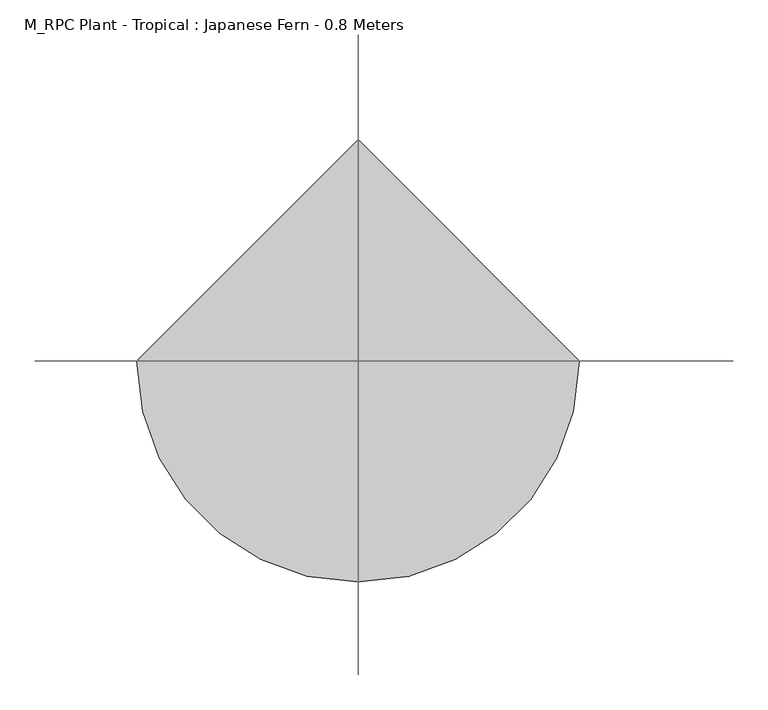
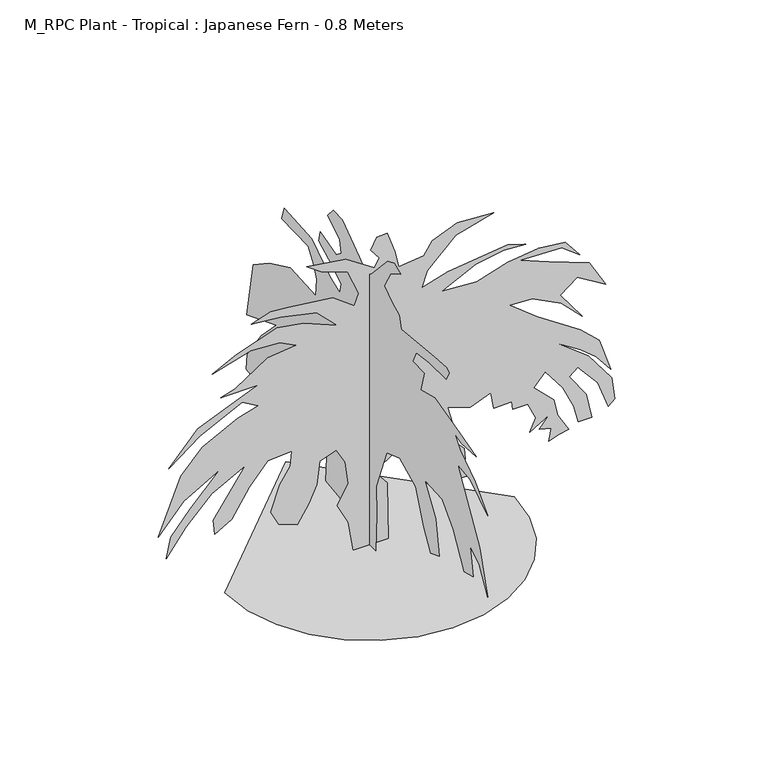
"""IFC4 building model written with IfcOpenShell, lengths in millimetres: geographic element geometry, M_RPC Plant - Tropical : Japanese Fern - 0.8 Meters."""

import ifcopenshell
import ifcopenshell.guid

model = None  # the IFC model being written
_history = None  # IfcOwnerHistory: only IFC2X3 demands one
_inside = {}  # id of a spatial element -> (the spatial element, [elements in it])
_under = {}  # id of a project, library or spatial element -> (it, [spatial elements below it])
_declared = {}  # id of a project -> (the project, [libraries it declares])
_typed = {}  # id of a type object -> (the type object, [elements of that type])
_made_of = {}  # id of a material, layer set ... -> (it, [elements and type objects made of it])


def new_model(schema):
    """Start an empty IFC model of exactly this schema.

    Asked for "IFC4X3", IfcOpenShell would pick the latest addendum, in which some entities
    have other attributes; the version numbers below select the first issue.
    IFC2X3 requires an IfcOwnerHistory on every rooted entity: one is made here for all.
    """
    global model, _history
    if schema == "IFC4X3":
        model = ifcopenshell.file(schema_version=(4, 3, 0, 0))
    else:
        model = ifcopenshell.file(schema=schema)
    _inside.clear()
    _under.clear()
    _declared.clear()
    _typed.clear()
    _made_of.clear()
    _history = None
    if model.schema == "IFC2X3":
        org = make("IfcOrganization", Name="unknown")
        user = make(
            "IfcPersonAndOrganization",
            ThePerson=make("IfcPerson", FamilyName="unknown"),
            TheOrganization=org,
        )
        app = make(
            "IfcApplication",
            ApplicationDeveloper=org,
            Version="unknown",
            ApplicationFullName="unknown",
            ApplicationIdentifier="unknown",
        )
        _history = make(
            "IfcOwnerHistory",
            OwningUser=user,
            OwningApplication=app,
            ChangeAction="ADDED",
            CreationDate=0,
        )
    return model


def make(cls, **values):
    """One entity of the class cls with the attributes given. An attribute that is None is left unset."""
    return model.create_entity(
        cls, **{name: value for name, value in values.items() if value is not None}
    )


def rooted(cls, **values):
    """An entity with a GlobalId (a new one), such as an element, a storey or a relation."""
    return make(cls, GlobalId=ifcopenshell.guid.new(), OwnerHistory=_history, **values)


def si_unit(unit_type, name, prefix=None):
    """IfcSIUnit, for example si_unit("LENGTHUNIT", "METRE", prefix="MILLI")."""
    return make("IfcSIUnit", UnitType=unit_type, Prefix=prefix, Name=name)


def assignment(units):
    """IfcUnitAssignment: the units of a project."""
    return None if units is None else make("IfcUnitAssignment", Units=units)


def point(xyz):
    """IfcCartesianPoint."""
    return None if xyz is None else make("IfcCartesianPoint", Coordinates=xyz)


def direction(xyz):
    """IfcDirection."""
    return None if xyz is None else make("IfcDirection", DirectionRatios=xyz)


def frame(location, z_axis=None, x_axis=None):
    """IfcAxis2Placement3D, a coordinate frame: its origin and axes. An axis left out is left unset."""
    return make(
        "IfcAxis2Placement3D",
        Location=point(location),
        Axis=direction(z_axis),
        RefDirection=direction(x_axis),
    )


def origin():
    """The frame at (0, 0, 0) with its axes left unset."""
    return frame((0.0, 0.0, 0.0))


def place(relative_to, where):
    """IfcLocalPlacement: puts the frame where relative to a parent placement (None: the world)."""
    return make(
        "IfcLocalPlacement", PlacementRelTo=relative_to, RelativePlacement=where
    )


def context(
    kind, dimensions, precision=None, world=None, true_north=None, identifier=None
):
    """IfcGeometricRepresentationContext, for example the 3D "Model" context."""
    return make(
        "IfcGeometricRepresentationContext",
        ContextIdentifier=identifier,
        ContextType=kind,
        CoordinateSpaceDimension=dimensions,
        Precision=precision,
        WorldCoordinateSystem=world,
        TrueNorth=true_north,
    )


def project(units=None, contexts=None):
    """IfcProject with its units and contexts."""
    return rooted(
        "IfcProject",
        Name="project",
        RepresentationContexts=contexts,
        UnitsInContext=assignment(units),
    )


def spatial(cls, under=None, at=None, **own):
    """A site, building, storey or space (cls), placed at a placement, below another one or the project."""
    s = rooted(cls, ObjectPlacement=at, **own)
    if under is not None:
        _under.setdefault(under.id(), (under, []))[1].append(s)
    return s


def point_list(points):
    """IfcCartesianPointList2D or 3D."""
    cls = (
        "IfcCartesianPointList2D" if len(points[0]) == 2 else "IfcCartesianPointList3D"
    )
    return make(cls, CoordList=points)


def triangles(points, corners, closed=None, point_numbers=None):
    """IfcTriangulatedFaceSet: each triangle names its three corners, points numbered from 1."""
    return make(
        "IfcTriangulatedFaceSet",
        Coordinates=point_list(points),
        Closed=closed,
        CoordIndex=corners,
        PnIndex=point_numbers,
    )


def shape(context_of_items, identifier, shape_type, items):
    """IfcShapeRepresentation: the items that make up one representation, for example the "Body"."""
    return make(
        "IfcShapeRepresentation",
        ContextOfItems=context_of_items,
        RepresentationIdentifier=identifier,
        RepresentationType=shape_type,
        Items=items,
    )


def source(mapping_origin, context_of_items, identifier, shape_type, items):
    """IfcRepresentationMap: a shape defined once, which mapped items show again and again."""
    return make(
        "IfcRepresentationMap",
        MappingOrigin=mapping_origin,
        MappedRepresentation=shape(context_of_items, identifier, shape_type, items),
    )


def transform(
    local_origin,
    x_axis=None,
    y_axis=None,
    z_axis=None,
    scale=None,
    scale2=None,
    scale3=None,
    uniform=True,
):
    """IfcCartesianTransformationOperator3D, or its non-uniform kind. x_axis, y_axis, z_axis: its Axis1, 2, 3."""
    if uniform:
        return make(
            "IfcCartesianTransformationOperator3D",
            Axis1=direction(x_axis),
            Axis2=direction(y_axis),
            LocalOrigin=point(local_origin),
            Scale=scale,
            Axis3=direction(z_axis),
        )
    return make(
        "IfcCartesianTransformationOperator3DnonUniform",
        Axis1=direction(x_axis),
        Axis2=direction(y_axis),
        LocalOrigin=point(local_origin),
        Scale=scale,
        Axis3=direction(z_axis),
        Scale2=scale2,
        Scale3=scale3,
    )


def mapped(mapping_source, mapping_target):
    """IfcMappedItem: shows the shape of a source again, moved by a transform."""
    return make(
        "IfcMappedItem", MappingSource=mapping_source, MappingTarget=mapping_target
    )


def made_of(thing, what):
    """Note that an element or type object is made of a material, layer set ...; save() writes the relation."""
    if what is not None:
        _made_of.setdefault(what.id(), (what, []))[1].append(thing)
    return thing


def element(
    cls,
    number,
    at=None,
    inside=None,
    cuts=None,
    type_object=None,
    material=None,
    context=None,
    identifier="Body",
    shape_type=None,
    held_by="IfcProductDefinitionShape",
    body=None,
    shapes=None,
    **own,
):
    """One element of the class cls, such as IfcWall. Its Tag is "e" and its number.

    at: its placement. inside: the storey or other place that contains it. cuts: it is an
    opening in that element (IfcRelVoidsElement). A single representation is given by context,
    identifier, shape_type and body (its items); several are given by shapes. held_by: the class
    of the entity that holds the representations. save() writes the other relations.
    """
    e = rooted(cls, Tag="e%d" % number, ObjectPlacement=at, **own)
    if body is not None:
        shapes = [shape(context, identifier, shape_type, body)]
    if shapes is not None:
        e.Representation = make(held_by, Representations=shapes)
    if inside is not None:
        _inside.setdefault(inside.id(), (inside, []))[1].append(e)
    if cuts is not None:
        rooted(
            "IfcRelVoidsElement", RelatingBuildingElement=cuts, RelatedOpeningElement=e
        )
    if type_object is not None:
        _typed.setdefault(type_object.id(), (type_object, []))[1].append(e)
    return made_of(e, material)


def aggregate(whole, parts):
    """IfcRelAggregates: a whole, such as a stair, and the parts it consists of."""
    return rooted("IfcRelAggregates", RelatingObject=whole, RelatedObjects=parts)


def save(model, path):
    """Write the relations noted so far, then the file.

    IfcRelAggregates (storeys below a building ...), IfcRelContainedInSpatialStructure (elements
    in a storey), IfcRelDefinesByType, IfcRelAssociatesMaterial and IfcRelDeclares: one each for
    every whole, place, type object, material and project.
    """
    for whole, parts in _under.values():
        aggregate(whole, parts)
    for where, things in _inside.values():
        rooted(
            "IfcRelContainedInSpatialStructure",
            RelatedElements=things,
            RelatingStructure=where,
        )
    for kind, things in _typed.values():
        rooted("IfcRelDefinesByType", RelatedObjects=things, RelatingType=kind)
    for what, things in _made_of.values():
        rooted("IfcRelAssociatesMaterial", RelatedObjects=things, RelatingMaterial=what)
    for by, libraries in _declared.values():
        rooted("IfcRelDeclares", RelatingContext=by, RelatedDefinitions=libraries)
    model.write(path)


def m_rpc_plant_tropical_japanese_fern_0_8_meters_89f61e38(model_context):
    return source(origin(), model_context, "Body", "Tessellation", [
        triangles([(-356.9816259, 0.0, 2.46e-05), (-347.538961, -81.8417886, 2.46e-05), (-320.6483422, -157.0003733, 2.46e-05), (-278.4590569, -223.3224515, 2.46e-05), (-223.1257884, -278.6557201, 2.46e-05), (-156.8037101, -320.8450235, 2.46e-05), (-81.6451164, -347.7356423, 2.46e-05), (0.1966867, -357.1783072, 2.46e-05), (82.0384609, -347.7356423, 2.46e-05), (157.1970364, -320.8450235, 2.46e-05), (223.5191146, -278.6557201, 2.46e-05), (278.8523832, -223.3224515, 2.46e-05), (321.0417048, -157.0003733, 2.46e-05), (347.9323236, -81.8417886, 2.46e-05), (357.3749886, 3.12e-05, 2.46e-05), (0.1966242, 357.1783072, 2.46e-05), (-39.591288, 2.4e-05, 3.8e-06), (-52.3886082, 2.53e-05, 77.2092589), (-79.4701856, 2.33e-05, 129.9044073), (-51.8286088, 1.92e-05, 179.0246285), (-59.6237998, 1.61e-05, 237.2005651), (-81.0099172, 1.47e-05, 275.3224025), (-121.8640096, 1.74e-05, 260.7322683), (-129.4650627, 2.12e-05, 202.3781994), (-150.0026445, 2.47e-05, 159.3985009), (-177.3082362, 2.85e-05, 114.8257492), (-224.1652416, 2.95e-05, 132.5502668), (-243.9444304, 2.81e-05, 171.1790318), (-221.0799103, 2.33e-05, 234.4691003), (-195.0511394, 1.98e-05, 273.6130591), (-191.2119478, 1.74e-05, 311.3276902), (-250.2614867, 2.02e-05, 307.4210246), (-296.6350369, 2.54e-05, 254.2280142), (-339.5123071, 3.14e-05, 185.9592888), (-381.4722822, 3.47e-05, 161.1515734), (-385.2696158, 3.25e-05, 199.7619347), (-305.7070304, 2.23e-05, 313.25835), (-389.2322737, 2.86e-05, 269.5890678), (-451.6135314, 3.51e-05, 205.2877965), (-501.5068159, 4.12e-05, 139.8979924), (-490.5788492, 3.76e-05, 191.9816683), (-441.6242065, 3.21e-05, 249.0544201), (-368.8616057, 2.43e-05, 325.6103577), (-458.3148665, 3.13e-05, 274.3943886), (-521.6481374, 3.83e-05, 202.3696607), (-465.4295122, 2.75e-05, 342.7516442), (-412.306919, 2.18e-05, 399.0182679), (-325.1523188, 1.53e-05, 444.1942168), (-273.6057376, 1.22e-05, 459.1648873), (-314.0723265, 1.26e-05, 482.4155394), (-418.6162359, 2.03e-05, 430.012924), (-495.2054927, 2.71e-05, 372.3782879), (-423.1042251, 1.92e-05, 451.5675676), (-315.4003341, 1.18e-05, 496.7035117), (-275.4804052, 9.1e-06, 512.7808371), (-366.2136206, 1.31e-05, 512.5835017), (-331.2056557, 1.09e-05, 523.2341598), (-250.2614867, 4.2e-06, 575.8901027), (-180.8079499, 7e-07, 584.7194329), (-221.0799103, 1.2e-06, 605.0713883), (-292.4937199, 4.1e-06, 609.4207232), (-387.4135983, 9.9e-06, 581.7274281), (-328.4856545, 5.5e-06, 612.0154049), (-227.295374, -1e-06, 646.7967121), (-161.5869029, -3.2e-06, 635.7193359), (-78.621382, -4.8e-06, 600.674055), (-129.4533356, -5.6e-06, 651.5887161), (-219.3260566, -2.8e-06, 670.7326784), (-291.1150432, -1e-07, 678.0232944), (-243.6241556, -3.1e-06, 694.5326792), (-199.2876722, -4.8e-06, 690.5139565), (-89.7989701, -8.8e-06, 676.7513517), (-37.2379591, -8.7e-06, 637.1700468), (-25.5654385, -1.1e-05, 666.3513325), (-53.2067405, -1.36e-05, 730.9165775), (-118.8594782, -1.21e-05, 754.0578976), (-153.9631858, -1.22e-05, 780.1592113), (-58.1566019, -1.55e-05, 766.6525503), (12.3701786, -1.58e-05, 718.8793036), (24.5030987, -1.76e-05, 741.3032982), (3.6158409, -1.84e-05, 768.4872494), (18.7047597, -2.07e-05, 796.1618683), (43.7640938, -2.19e-05, 798.4898512), (62.816342, -1.95e-05, 744.3539114), (72.129132, -1.74e-05, 701.4126371), (134.0245409, -2.04e-05, 707.8552671), (155.3583768, -2.33e-05, 739.3059637), (216.6393747, -2.75e-05, 765.5672241), (307.1003683, -3.11e-05, 759.7325512), (213.1465828, -2.54e-05, 733.5272467), (143.1669335, -1.83e-05, 665.9780268), (130.1258781, -1.53e-05, 625.1620588), (193.29407, -1.93e-05, 645.9246723), (342.1190157, -2.69e-05, 663.433996), (386.0096143, -2.8e-05, 650.2686659), (331.6310294, -2.58e-05, 653.215361), (262.3572055, -2.2e-05, 640.2313425), (179.4618111, -1.6e-05, 599.1567421), (265.035058, -1.94e-05, 594.3860667), (342.0896934, -2.42e-05, 617.5967503), (417.9909471, -2.81e-05, 628.4153486), (483.3268573, -3.05e-05, 620.5620489), (520.1241752, -2.95e-05, 575.8901027), (475.7348788, -2.95e-05, 609.4687217), (372.9456588, -2.52e-05, 612.3860945), (441.3349073, -2.65e-05, 584.6447645), (542.8041498, -2.87e-05, 546.4048021), (584.2227699, -2.63e-05, 476.0742113), (513.9028253, -2.58e-05, 519.0714778), (472.0308898, -2.2e-05, 486.8048427), (525.9615005, -2e-05, 412.4742416), (473.4335295, -2.08e-05, 465.0022127), (402.3962957, -1.99e-05, 501.5674953), (346.6470097, -1.76e-05, 504.9195073), (415.0709218, -1.74e-05, 450.4102255), (520.5801793, -1.78e-05, 379.9196154), (568.2414416, -1.72e-05, 335.1356847), (596.0814211, -1.33e-05, 249.2213612), (560.7561427, -1.45e-05, 294.909034), (522.6121774, -1.47e-05, 326.2076686), (462.342891, -1.43e-05, 363.9543108), (540.550799, -1.42e-05, 304.5037063), (599.2467439, -1.21e-05, 226.7565805), (605.6067481, -9e-06, 169.6256927), (590.1587448, -7.5e-06, 155.6795782), (563.8974481, -1.05e-05, 225.714711), (514.2895022, -1.18e-05, 284.0770462), (493.1588516, -9.9e-06, 266.7677284), (536.2361641, -8.1e-06, 205.2771322), (549.3054608, -4.8e-06, 141.0889262), (516.425491, -3.3e-06, 140.2646579), (505.3241701, -5.5e-06, 185.108614), (477.6415575, -7.8e-06, 243.2032329), (434.3535748, -9.2e-06, 299.3437015), (405.9722766, -6.1e-06, 268.3197412), (455.9268946, -5.4e-06, 219.8784575), (465.4788915, -3.2e-06, 174.9152863), (492.2202098, -1.7e-06, 130.1460077), (468.8415496, -3e-07, 124.1884135), (442.7215596, 1.3e-06, 116.1070845), (449.5455617, -8e-07, 146.8782531), (419.662938, 0.0, 155.0435705), (444.2522438, -2.8e-06, 184.860882), (396.2229444, 1e-06, 156.0027779), (410.9322573, -1.6e-06, 188.0872839), (391.7616251, -3.2e-06, 229.804832), (353.6443296, -1.6e-06, 230.0109786), (351.7750033, -2.7e-06, 250.1848198), (307.1003683, -7e-07, 249.0597613), (300.2817075, -2.9e-06, 291.6023862), (248.7385418, 5e-07, 272.405066), (193.29407, 1.9e-06, 289.9143715), (210.8028487, 4.9e-06, 225.714711), (209.5596469, 6.7e-06, 196.5163297), (234.147899, 7.2e-06, 170.2702392), (237.0660348, 8.8e-06, 141.0889262), (219.1519212, 1.04e-05, 127.6382756), (249.9017521, 1.1e-05, 94.9585752), (191.3132679, 1.34e-05, 97.4711035), (201.263133, 1.05e-05, 139.9955973), (173.9058276, 1.05e-05, 159.8089046), (182.4415529, 8.6e-06, 185.1459482), (114.684288, 1.2e-05, 178.0643492), (99.9141775, 1.12e-05, 202.3696607), (152.4405135, 7.1e-06, 231.5509645), (87.6747175, 9.8e-06, 234.8944377), (12.4554318, 1.6e-05, 186.0566121), (44.4696966, 1.69e-05, 146.9251888), (47.3878233, 1.91e-05, 0.0), (0.1988968, 28.0250381, 3.7e-06), (0.1989024, 23.3153101, 131.4809371), (0.1989043, 63.1703357, 135.2526637), (0.1989031, 125.3580096, 45.104755), (0.1989061, 186.8720783, 53.6724779), (0.1989088, 182.1083611, 118.7774792), (0.1989112, 144.4259864, 212.5160617), (0.1989072, 143.3849253, 265.1541278), (0.1989091, 175.7563505, 275.9837175), (0.1989147, 237.6858916, 199.7619347), (0.198915, 302.7357001, 140.1214617), (0.1989165, 331.3730146, 147.3601187), (0.1989186, 325.3463476, 199.5424713), (0.1989213, 363.9222997, 223.1101825), (0.1989223, 429.8262348, 180.7067569), (0.1989222, 475.8741872, 131.4809371), (0.1989247, 526.6901261, 139.4206596), (0.1989263, 521.9248283, 180.7067569), (0.1989212, 463.1728912, 264.866936), (0.1989213, 397.7889462, 332.7090159), (0.1989246, 523.5141572, 283.9223863), (0.1989299, 495.7835097, 430.9862294), (0.1989289, 428.236906, 476.0608764), (0.1989268, 339.3143177, 517.3488358), (0.1989217, 228.4952462, 512.2821756), (0.1989235, 224.9824519, 557.0447777), (0.1989254, 238.2328241, 586.9834299), (0.198928, 261.7722666, 621.3780602), (0.198933, 375.8342906, 623.7380178), (0.198934, 364.7196347, 657.0846743), (0.1989285, 247.1213622, 649.612674), (0.1989229, 169.3534347, 598.4660866), (0.1989203, 125.6708085, 581.7007582), (0.1989213, 121.2033486, 608.4554114), (0.1989249, 174.1686204, 639.6180079), (0.1989278, 217.0427113, 661.8500084), (0.1989224, 209.1029888, 690.4313307), (0.1989186, 140.9505263, 671.9353666), (0.1989184, 120.1790834, 688.8446543), (0.1989201, 126.4332074, 719.3166315), (0.1989238, 178.9323558, 752.3619255), (0.1989239, 155.1134427, 779.3565714), (0.1989222, 117.0030872, 777.7672062), (0.1989167, 43.7690217, 725.5806387), (0.1989142, 11.282335, 699.1806513), (0.1989139, -10.6222293, 714.4366241), (0.1989141, -78.3121894, 787.2951857), (0.1989134, -106.8948288, 799.9992067), (0.1989117, -133.8897381, 787.2951857), (0.1989124, -91.4905729, 762.6498877), (0.1989115, -63.82447, 714.9192982), (0.198909, -97.1412363, 690.3886734), (0.1989071, -127.8788042, 676.3806622), (0.1989116, -136.2243976, 645.8900087), (0.1988998, -278.3917282, 660.2606432), (0.1988976, -330.7943436, 663.4366848), (0.1988968, -341.9089994, 655.4979979), (0.1989026, -329.2050147, 631.6793936), (0.1989057, -255.7989394, 630.9247158), (0.1989078, -201.4115251, 623.4394169), (0.1989071, -185.4035451, 591.3727332), (0.1989049, -234.4786928, 590.4820899), (0.1989033, -219.4389858, 537.8608106), (0.1989013, -279.9783864, 553.8714612), (0.1988956, -384.8262926, 526.9594774), (0.1988915, -456.2395572, 506.2314912), (0.1988942, -394.0155936, 503.9995053), (0.1988957, -365.7943148, 511.6901696), (0.1988935, -388.4636069, 482.6261733), (0.1988888, -452.284893, 439.6635704), (0.198884, -507.0528437, 383.9622828), (0.1988894, -430.8768974, 431.8128868), (0.198892, -378.3489627, 438.6928811), (0.1988872, -418.3222495, 368.7036212), (0.1988809, -472.1195472, 279.1570521), (0.1988809, -505.8634904, 170.2702392), (0.198879, -470.530182, 233.1083004), (0.1988817, -430.9435721, 256.6434736), (0.1988781, -444.5382365, 186.5443548), (0.1988855, -406.6475987, 176.1064927), (0.198885, -359.3756295, 258.5152162), (0.1988892, -311.2476806, 308.3676965), (0.1988927, -237.3971011, 313.25835), (0.1988874, -284.7437206, 241.0480229), (0.1988892, -298.5170441, 151.7734485), (0.1988901, -261.8053315, 136.5182659), (0.1988937, -232.8570984, 188.3064747), (0.1988926, -197.5672648, 272.0370652), (0.198897, -130.1718691, 304.5676922), (0.1988986, -73.5660583, 284.6663815), (0.1989018, -28.8695723, 170.457437), (0.1988986, -31.953834, 99.3204365), (0.1988944, -26.9829074, 2.55e-05)], [[15, 16, 1], [14, 15, 1], [14, 1, 2], [13, 14, 2], [13, 2, 3], [13, 3, 4], [12, 13, 4], [11, 12, 4], [11, 4, 5], [11, 5, 6], [11, 6, 7], [11, 7, 8], [11, 8, 9], [11, 9, 10], [110, 111, 112], [51, 52, 53], [61, 62, 63], [102, 103, 104], [94, 95, 96], [55, 56, 57], [88, 89, 90], [44, 45, 46], [117, 118, 119], [61, 63, 64], [68, 69, 70], [39, 40, 41], [107, 108, 109], [76, 77, 78], [39, 41, 42], [75, 76, 78], [38, 39, 42], [38, 42, 43], [60, 61, 64], [143, 144, 145], [93, 94, 96], [93, 96, 97], [93, 97, 98], [68, 70, 71], [37, 38, 43], [55, 57, 58], [157, 158, 159], [157, 159, 160], [75, 78, 79], [92, 93, 98], [74, 75, 79], [67, 68, 71], [67, 71, 72], [110, 112, 113], [139, 140, 141], [87, 88, 90], [87, 90, 91], [86, 87, 91], [117, 119, 120], [116, 117, 120], [116, 120, 121], [115, 116, 121], [101, 102, 104], [101, 104, 105], [100, 101, 105], [106, 107, 109], [34, 35, 36], [141, 142, 143], [43, 44, 46], [43, 46, 47], [124, 125, 126], [123, 124, 126], [122, 123, 126], [122, 126, 127], [34, 36, 37], [33, 34, 37], [32, 33, 37], [60, 64, 65], [59, 60, 65], [137, 138, 139], [137, 139, 141], [137, 141, 143], [136, 137, 143], [121, 122, 127], [50, 51, 53], [50, 53, 54], [66, 67, 72], [66, 72, 73], [106, 109, 110], [106, 110, 113], [129, 130, 131], [129, 131, 132], [129, 132, 133], [128, 129, 133], [128, 133, 134], [43, 47, 48], [37, 43, 48], [105, 106, 113], [105, 113, 114], [100, 105, 114], [99, 100, 114], [59, 65, 66], [163, 164, 165], [162, 163, 165], [168, 169, 17], [168, 17, 18], [168, 18, 19], [168, 19, 20], [167, 168, 20], [167, 20, 21], [146, 147, 148], [121, 127, 128], [121, 128, 134], [85, 86, 91], [148, 149, 150], [37, 48, 49], [32, 37, 49], [31, 32, 49], [85, 91, 92], [25, 26, 27], [25, 27, 28], [25, 28, 29], [24, 25, 29], [24, 29, 30], [23, 24, 30], [23, 30, 31], [136, 143, 145], [135, 136, 145], [135, 145, 146], [135, 146, 148], [82, 83, 84], [81, 82, 84], [80, 81, 84], [80, 84, 85], [79, 80, 85], [50, 54, 55], [49, 50, 55], [160, 161, 162], [156, 157, 160], [155, 156, 160], [155, 160, 162], [154, 155, 162], [154, 162, 165], [153, 154, 165], [152, 153, 165], [74, 79, 85], [74, 85, 92], [73, 74, 92], [166, 167, 21], [55, 58, 59], [166, 21, 22], [152, 165, 166], [135, 148, 150], [134, 135, 150], [121, 134, 150], [115, 121, 150], [114, 115, 150], [114, 150, 151], [114, 151, 152], [99, 114, 152], [98, 99, 152], [98, 152, 166], [98, 166, 22], [92, 98, 22], [73, 92, 22], [66, 73, 22], [59, 66, 22], [55, 59, 22], [49, 55, 22], [31, 49, 22], [23, 31, 22], [244, 245, 246], [239, 240, 241], [234, 235, 236], [234, 236, 237], [233, 234, 237], [238, 239, 241], [238, 241, 242], [217, 218, 219], [216, 217, 219], [189, 190, 191], [244, 246, 247], [215, 216, 219], [215, 219, 220], [197, 198, 199], [197, 199, 200], [230, 231, 232], [189, 191, 192], [209, 210, 211], [209, 211, 212], [209, 212, 213], [208, 209, 213], [197, 200, 201], [196, 197, 201], [195, 196, 201], [243, 244, 247], [262, 170, 171], [261, 262, 171], [260, 261, 171], [205, 206, 207], [204, 205, 207], [203, 204, 207], [185, 186, 187], [184, 185, 187], [184, 187, 188], [183, 184, 188], [183, 188, 189], [173, 174, 175], [172, 173, 175], [172, 175, 176], [247, 248, 249], [247, 249, 250], [243, 247, 250], [243, 250, 251], [242, 243, 251], [254, 255, 256], [253, 254, 256], [253, 256, 257], [252, 253, 257], [225, 226, 227], [224, 225, 227], [224, 227, 228], [223, 224, 228], [223, 228, 229], [223, 229, 230], [180, 181, 182], [179, 180, 182], [189, 192, 193], [189, 193, 194], [252, 257, 258], [203, 207, 208], [242, 251, 252], [208, 213, 214], [203, 208, 214], [183, 189, 194], [182, 183, 194], [179, 182, 194], [178, 179, 194], [177, 178, 194], [195, 201, 202], [194, 195, 202], [177, 194, 202], [237, 238, 242], [237, 242, 252], [233, 237, 252], [232, 233, 252], [232, 252, 258], [230, 232, 258], [230, 258, 259], [223, 230, 259], [221, 222, 223], [221, 223, 259], [220, 221, 259], [215, 220, 259], [214, 215, 259], [203, 214, 259], [202, 203, 259], [177, 202, 259], [177, 259, 260], [176, 177, 260], [172, 176, 260], [172, 260, 171]], closed=False),
    ])


if __name__ == "__main__":
    model = new_model("IFC4")
    model_context = context("Model", 3, world=origin())
    ifc_project = project(units=[si_unit("LENGTHUNIT", "METRE", prefix="MILLI")], contexts=[model_context])
    site = spatial("IfcSite", under=ifc_project)
    building = spatial("IfcBuilding", under=site)
    placement = place(None, origin())
    m_rpc_plant_tropical_japanese_fern_0_8_meters_shape = m_rpc_plant_tropical_japanese_fern_0_8_meters_89f61e38(model_context)
    element("IfcGeographicElement", 1, ObjectType="M_RPC Plant - Tropical : Japanese Fern - 0.8 Meters", at=placement, inside=building, context=model_context, shape_type="MappedRepresentation", body=[
        mapped(m_rpc_plant_tropical_japanese_fern_0_8_meters_shape, transform((0.0, 0.0, 0.0), x_axis=(1.0, 0.0, 0.0), y_axis=(0.0, 1.0, 0.0), z_axis=(0.0, 0.0, 1.0))),
    ])
    save(model, "model.ifc")

# Revit data of these elements
# Type "M_RPC Plant - Tropical : Japanese Fern - 0.8 Meters"
#   built-in parameter 1005198 = "{2, 15},{39, RPC-16-G1GK-JAPX-7J4P-Q000-ST1L-LVER-AU},{1, 0},{1, 0},{2, 35},{1, 8},{5, Color},{1, 0},{1, 0},{3, 0.8},{3, 0.8},{3, 0.8},{1, 8},{7, BBoxMin},{1, 0},{1, 0},{1, 0},{1, 0},{1, 0},{1, 8},{7, BBoxMax},{1, 0},{1, 0},{1, 0},{1, 0},{1, 0},{2, 11},{9, RPCTypeId},{1, 0},{1, 0},{39, RPC-16-G1GK-JAPX-7J4P-Q000-ST1L-LVER-AU},{1, 6},{14, RPCPlantHeight},{1, 0},{1, 0},{7, 2.62467},{2, 11},{7, keyword},{1, 0},{1, 0},{53, :Geometry:RPC:Japanese Fern:plant:small:japanese fern},{2, 11},{8, category},{1, 0},{1, 0},{17, :Shrubs [General]},{2, 11},{12, LocalizedUID},{1, 0},{1, 0},{13, Japanese Fern},{2, 14},{6, Height},{1, 0},{1, 0},{7, 2.62467},{1, 2},{16, Cast Reflections},{1, 0},{1, 0},{1, 0},{1, 2},{12, Cast Shadows},{1, 0},{1, 0},{1, 1},{1, 2},{9, Lock View},{1, 0},{1, 0},{1, 0},{1, 4},{5, ViewC},{1, 0},{1, 0},{1, 0},{2, 11},{20, AdvancedUIDefinition},{1, 0},{1, 0},{0, },{2, 11},{10, AssetLibID},{1, 0},{1, 0},{36, 4D3F6E72-3F99-4203-98E9-AF80B3C7A7A4},{2, 11},{10, BaseSchema},{1, 0},{1, 0},{9, RPCSchema},{2, 11},{12, ExchangeGUID},{1, 0},{1, 0},{0, },{1, 2},{6, Hidden},{1, 0},{1, 0},{1, 0},{1, 4},{11, RPCCategory},{1, 0},{1, 0},{1, 0},{2, 11},{8, RPCImage},{1, 0},{1, 0},{0, },{1, 4},{13, SchemaVersion},{1, 0},{1, 0},{1, 4},{2, 11},{12, UIDefinition},{1, 0},{1, 0},{0, },{2, 11},{6, UIName},{1, 0},{1, 0},{39, RPC-16-G1GK-JAPX-7J4P-Q000-ST1L-LVER-AU},{2, 11},{11, VersionGUID},{1, 0},{1, 0},{9, RPCSchema},{2, 11},{9, assettype},{1, 0},{1, 0},{11, RPCGeometry},{2, 11},{11, description},{1, 0},{1, 0},{0, },{2, 11},{9, localname},{1, 0},{1, 0},{3, RPC},{2, 11},{9, localtype},{1, 0},{1, 0},{3, RPC},{1, 4},{8, revision},{1, 0},{1, 0},{1, 1},{2, 11},{9, thumbnail},{1, 0},{1, 0},{0, },{1, 4},{7, version},{1, 0},{1, 0},{1, 1},{1, 2},{20, RPC_Cast Reflections},{1, 0},{1, 0},{1, 1},{1, 2},{16, RPC_Cast Shadows},{1, 0},{1, 0},{1, 1},{1, 2},{13, RPC_Lock View},{1, 0},{1, 0},{1, 0},{1, 4},{9, RPC_ViewC},{1, 0},{1, 0},{1, 0},{21, assetlibrary_base.fbx},{1, 5},"
#   built-in parameter 1005195 = "RPC-16-G1GK-JAPX-7J4P-Q000-ST1L-LVER-AU"
#   Type Comments = "Japanese Fern"
#   Height = 0.8 m
#   Description = (empty or 0)
#   Default Elevation = 0
